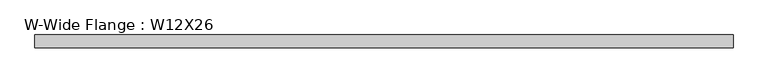
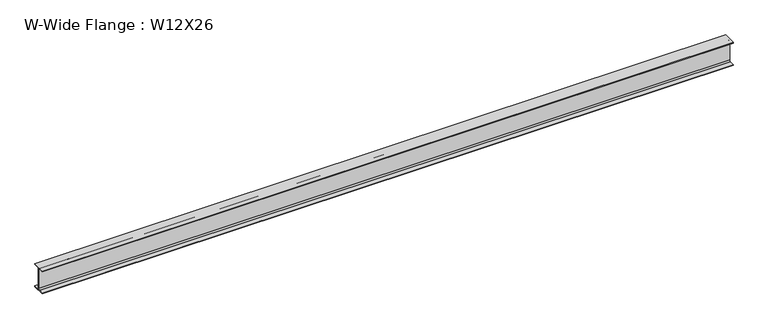
"""IFC4 building model written with IfcOpenShell, lengths in millimetres: beam geometry, W-Wide Flange : W12X26."""

import ifcopenshell
import ifcopenshell.guid

model = None  # the IFC model being written
_history = None  # IfcOwnerHistory: only IFC2X3 demands one
_inside = {}  # id of a spatial element -> (the spatial element, [elements in it])
_under = {}  # id of a project, library or spatial element -> (it, [spatial elements below it])
_declared = {}  # id of a project -> (the project, [libraries it declares])
_typed = {}  # id of a type object -> (the type object, [elements of that type])
_made_of = {}  # id of a material, layer set ... -> (it, [elements and type objects made of it])


def new_model(schema):
    """Start an empty IFC model of exactly this schema.

    Asked for "IFC4X3", IfcOpenShell would pick the latest addendum, in which some entities
    have other attributes; the version numbers below select the first issue.
    IFC2X3 requires an IfcOwnerHistory on every rooted entity: one is made here for all.
    """
    global model, _history
    if schema == "IFC4X3":
        model = ifcopenshell.file(schema_version=(4, 3, 0, 0))
    else:
        model = ifcopenshell.file(schema=schema)
    _inside.clear()
    _under.clear()
    _declared.clear()
    _typed.clear()
    _made_of.clear()
    _history = None
    if model.schema == "IFC2X3":
        org = make("IfcOrganization", Name="unknown")
        user = make(
            "IfcPersonAndOrganization",
            ThePerson=make("IfcPerson", FamilyName="unknown"),
            TheOrganization=org,
        )
        app = make(
            "IfcApplication",
            ApplicationDeveloper=org,
            Version="unknown",
            ApplicationFullName="unknown",
            ApplicationIdentifier="unknown",
        )
        _history = make(
            "IfcOwnerHistory",
            OwningUser=user,
            OwningApplication=app,
            ChangeAction="ADDED",
            CreationDate=0,
        )
    return model


def make(cls, **values):
    """One entity of the class cls with the attributes given. An attribute that is None is left unset."""
    return model.create_entity(
        cls, **{name: value for name, value in values.items() if value is not None}
    )


def rooted(cls, **values):
    """An entity with a GlobalId (a new one), such as an element, a storey or a relation."""
    return make(cls, GlobalId=ifcopenshell.guid.new(), OwnerHistory=_history, **values)


def si_unit(unit_type, name, prefix=None):
    """IfcSIUnit, for example si_unit("LENGTHUNIT", "METRE", prefix="MILLI")."""
    return make("IfcSIUnit", UnitType=unit_type, Prefix=prefix, Name=name)


def assignment(units):
    """IfcUnitAssignment: the units of a project."""
    return None if units is None else make("IfcUnitAssignment", Units=units)


def point(xyz):
    """IfcCartesianPoint."""
    return None if xyz is None else make("IfcCartesianPoint", Coordinates=xyz)


def direction(xyz):
    """IfcDirection."""
    return None if xyz is None else make("IfcDirection", DirectionRatios=xyz)


def frame(location, z_axis=None, x_axis=None):
    """IfcAxis2Placement3D, a coordinate frame: its origin and axes. An axis left out is left unset."""
    return make(
        "IfcAxis2Placement3D",
        Location=point(location),
        Axis=direction(z_axis),
        RefDirection=direction(x_axis),
    )


def frame_2d(location, x_axis=None):
    """IfcAxis2Placement2D, a coordinate frame in the plane: its origin and x axis."""
    return make(
        "IfcAxis2Placement2D", Location=point(location), RefDirection=direction(x_axis)
    )


def origin():
    """The frame at (0, 0, 0) with its axes left unset."""
    return frame((0.0, 0.0, 0.0))


def place(relative_to, where):
    """IfcLocalPlacement: puts the frame where relative to a parent placement (None: the world)."""
    return make(
        "IfcLocalPlacement", PlacementRelTo=relative_to, RelativePlacement=where
    )


def context(
    kind, dimensions, precision=None, world=None, true_north=None, identifier=None
):
    """IfcGeometricRepresentationContext, for example the 3D "Model" context."""
    return make(
        "IfcGeometricRepresentationContext",
        ContextIdentifier=identifier,
        ContextType=kind,
        CoordinateSpaceDimension=dimensions,
        Precision=precision,
        WorldCoordinateSystem=world,
        TrueNorth=true_north,
    )


def project(units=None, contexts=None):
    """IfcProject with its units and contexts."""
    return rooted(
        "IfcProject",
        Name="project",
        RepresentationContexts=contexts,
        UnitsInContext=assignment(units),
    )


def spatial(cls, under=None, at=None, **own):
    """A site, building, storey or space (cls), placed at a placement, below another one or the project."""
    s = rooted(cls, ObjectPlacement=at, **own)
    if under is not None:
        _under.setdefault(under.id(), (under, []))[1].append(s)
    return s


def polyline(points):
    """IfcPolyline through the points."""
    return make("IfcPolyline", Points=[point(p) for p in points])


def circle_curve(where, radius):
    """IfcCircle in the frame where."""
    return make("IfcCircle", Position=where, Radius=radius)


def trimmed(basis, trim1, trim2, sense, master):
    """IfcTrimmedCurve: the piece of a basis curve between two trims."""
    return make(
        "IfcTrimmedCurve",
        BasisCurve=basis,
        Trim1=trim1,
        Trim2=trim2,
        SenseAgreement=sense,
        MasterRepresentation=master,
    )


def segment(curve, same_sense, transition):
    """IfcCompositeCurveSegment."""
    return make(
        "IfcCompositeCurveSegment",
        Transition=transition,
        SameSense=same_sense,
        ParentCurve=curve,
    )


def composite_curve(segments, self_intersect=None):
    """IfcCompositeCurve: segments joined end to end."""
    return make("IfcCompositeCurve", Segments=segments, SelfIntersect=self_intersect)


def outline(outer, holes=None, kind="AREA"):
    """IfcArbitraryClosedProfileDef: a profile drawn as a closed curve; with holes, ...WithVoids."""
    if holes is None:
        return make("IfcArbitraryClosedProfileDef", ProfileType=kind, OuterCurve=outer)
    return make(
        "IfcArbitraryProfileDefWithVoids",
        ProfileType=kind,
        OuterCurve=outer,
        InnerCurves=holes,
    )


def extrude(swept, where, along, depth):
    """IfcExtrudedAreaSolid: the profile swept, set in the frame where, extruded along a direction by depth."""
    return make(
        "IfcExtrudedAreaSolid",
        SweptArea=swept,
        Position=where,
        ExtrudedDirection=direction(along),
        Depth=depth,
    )


def shape(context_of_items, identifier, shape_type, items):
    """IfcShapeRepresentation: the items that make up one representation, for example the "Body"."""
    return make(
        "IfcShapeRepresentation",
        ContextOfItems=context_of_items,
        RepresentationIdentifier=identifier,
        RepresentationType=shape_type,
        Items=items,
    )


def source(mapping_origin, context_of_items, identifier, shape_type, items):
    """IfcRepresentationMap: a shape defined once, which mapped items show again and again."""
    return make(
        "IfcRepresentationMap",
        MappingOrigin=mapping_origin,
        MappedRepresentation=shape(context_of_items, identifier, shape_type, items),
    )


def transform(
    local_origin,
    x_axis=None,
    y_axis=None,
    z_axis=None,
    scale=None,
    scale2=None,
    scale3=None,
    uniform=True,
):
    """IfcCartesianTransformationOperator3D, or its non-uniform kind. x_axis, y_axis, z_axis: its Axis1, 2, 3."""
    if uniform:
        return make(
            "IfcCartesianTransformationOperator3D",
            Axis1=direction(x_axis),
            Axis2=direction(y_axis),
            LocalOrigin=point(local_origin),
            Scale=scale,
            Axis3=direction(z_axis),
        )
    return make(
        "IfcCartesianTransformationOperator3DnonUniform",
        Axis1=direction(x_axis),
        Axis2=direction(y_axis),
        LocalOrigin=point(local_origin),
        Scale=scale,
        Axis3=direction(z_axis),
        Scale2=scale2,
        Scale3=scale3,
    )


def mapped(mapping_source, mapping_target):
    """IfcMappedItem: shows the shape of a source again, moved by a transform."""
    return make(
        "IfcMappedItem", MappingSource=mapping_source, MappingTarget=mapping_target
    )


def made_of(thing, what):
    """Note that an element or type object is made of a material, layer set ...; save() writes the relation."""
    if what is not None:
        _made_of.setdefault(what.id(), (what, []))[1].append(thing)
    return thing


def element(
    cls,
    number,
    at=None,
    inside=None,
    cuts=None,
    type_object=None,
    material=None,
    context=None,
    identifier="Body",
    shape_type=None,
    held_by="IfcProductDefinitionShape",
    body=None,
    shapes=None,
    **own,
):
    """One element of the class cls, such as IfcWall. Its Tag is "e" and its number.

    at: its placement. inside: the storey or other place that contains it. cuts: it is an
    opening in that element (IfcRelVoidsElement). A single representation is given by context,
    identifier, shape_type and body (its items); several are given by shapes. held_by: the class
    of the entity that holds the representations. save() writes the other relations.
    """
    e = rooted(cls, Tag="e%d" % number, ObjectPlacement=at, **own)
    if body is not None:
        shapes = [shape(context, identifier, shape_type, body)]
    if shapes is not None:
        e.Representation = make(held_by, Representations=shapes)
    if inside is not None:
        _inside.setdefault(inside.id(), (inside, []))[1].append(e)
    if cuts is not None:
        rooted(
            "IfcRelVoidsElement", RelatingBuildingElement=cuts, RelatedOpeningElement=e
        )
    if type_object is not None:
        _typed.setdefault(type_object.id(), (type_object, []))[1].append(e)
    return made_of(e, material)


def aggregate(whole, parts):
    """IfcRelAggregates: a whole, such as a stair, and the parts it consists of."""
    return rooted("IfcRelAggregates", RelatingObject=whole, RelatedObjects=parts)


def save(model, path):
    """Write the relations noted so far, then the file.

    IfcRelAggregates (storeys below a building ...), IfcRelContainedInSpatialStructure (elements
    in a storey), IfcRelDefinesByType, IfcRelAssociatesMaterial and IfcRelDeclares: one each for
    every whole, place, type object, material and project.
    """
    for whole, parts in _under.values():
        aggregate(whole, parts)
    for where, things in _inside.values():
        rooted(
            "IfcRelContainedInSpatialStructure",
            RelatedElements=things,
            RelatingStructure=where,
        )
    for kind, things in _typed.values():
        rooted("IfcRelDefinesByType", RelatedObjects=things, RelatingType=kind)
    for what, things in _made_of.values():
        rooted("IfcRelAssociatesMaterial", RelatedObjects=things, RelatingMaterial=what)
    for by, libraries in _declared.values():
        rooted("IfcRelDeclares", RelatingContext=by, RelatedDefinitions=libraries)
    model.write(path)


def w_wide_flange_w12x26_21dbd052(model_context):
    return source(origin(), model_context, "Body", "SweptSolid", [
        extrude(outline(composite_curve([segment(polyline([(82.4011719, -145.5539063), (82.4011719, -155.178125), (-82.4011719, -155.178125), (-82.4011719, -145.5539063), (-20.2902344, -145.5539063)]), True, "CONTINUOUS"), segment(trimmed(circle_curve(frame_2d((-20.2902344, -128.190625)), 17.3632812), [point((-20.2902344, -145.5539063))], [point((-2.9269531, -128.190625))], True, "CARTESIAN"), True, "CONTINUOUS"), segment(polyline([(-2.9269531, -128.190625), (-2.9269531, 128.190625)]), True, "CONTINUOUS"), segment(trimmed(circle_curve(frame_2d((-20.2902344, 128.190625)), 17.3632812), [point((-2.9269531, 128.190625))], [point((-20.2902344, 145.5539062))], True, "CARTESIAN"), True, "CONTINUOUS"), segment(polyline([(-20.2902344, 145.5539062), (-82.4011719, 145.5539062), (-82.4011719, 155.178125), (82.4011719, 155.178125), (82.4011719, 145.5539062), (20.2902344, 145.5539062)]), True, "CONTINUOUS"), segment(trimmed(circle_curve(frame_2d((20.2902344, 128.190625)), 17.3632812), [point((20.2902344, 145.5539062))], [point((2.9269531, 128.190625))], True, "CARTESIAN"), True, "CONTINUOUS"), segment(polyline([(2.9269531, 128.190625), (2.9269531, -128.190625)]), True, "CONTINUOUS"), segment(trimmed(circle_curve(frame_2d((20.2902344, -128.190625)), 17.3632812), [point((2.9269531, -128.190625))], [point((20.2902344, -145.5539063))], True, "CARTESIAN"), True, "CONTINUOUS"), segment(polyline([(20.2902344, -145.5539063), (82.4011719, -145.5539063)]), True, "CONTINUOUS")], self_intersect=False)), frame((-3657.6, 0.0, 0.0), z_axis=(1.0, 0.0, 0.0), x_axis=(0.0, 1.0, 0.0)), (0.0, 0.0, 1.0), 8839.2),
    ])


if __name__ == "__main__":
    model = new_model("IFC4")
    model_context = context("Model", 3, world=origin())
    ifc_project = project(units=[si_unit("LENGTHUNIT", "METRE", prefix="MILLI")], contexts=[model_context])
    site = spatial("IfcSite", under=ifc_project)
    building = spatial("IfcBuilding", under=site)
    placement = place(None, origin())
    w_wide_flange_w12x26_shape = w_wide_flange_w12x26_21dbd052(model_context)
    element("IfcBeam", 1, ObjectType="W-Wide Flange : W12X26", at=placement, inside=building, context=model_context, shape_type="MappedRepresentation", body=[
        mapped(w_wide_flange_w12x26_shape, transform((0.0, 0.0, 0.0), x_axis=(1.0, 0.0, 0.0), y_axis=(0.0, 1.0, 0.0), z_axis=(0.0, 0.0, 1.0))),
    ])
    save(model, "model.ifc")

# Revit data of these elements
# Type "W-Wide Flange : W12X26"
#   Assembly Code = "B10"
#   W = 26
#   Length [instance default] = 5' - 0"
#   bf = 0' - 6 125/256"
#   d = 1' - 0 7/32"
#   k = 0' - 1 1/16"
#   k2 = 0' - 0 175/256"
#   tf = 0' - 0 97/256"
#   tw = 0' - 0 59/256"
#   A = 0.053125 SF
#   Structural Material [instance default] = none
